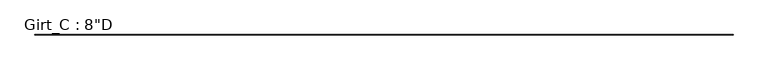
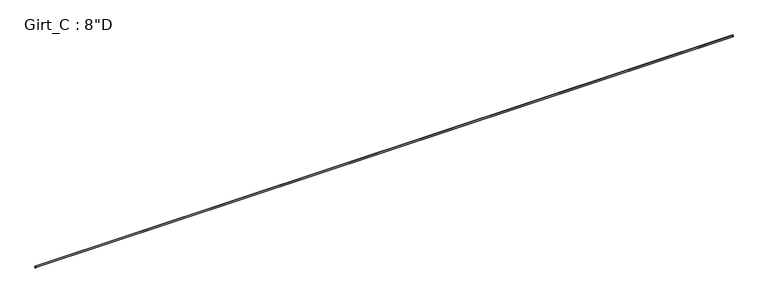
"""IFC4 building model written with IfcOpenShell, lengths in millimetres: beam geometry."""

from ifc_helpers import new_model, si_unit, point, frame, frame_2d, origin, place, context, project, spatial, polyline, circle_curve, trimmed, segment, composite_curve, outline, extrude, source, transform, mapped, element, save


def beam_1fd13926(model_context):
    return source(origin(), model_context, "Body", "SweptSolid", [
        extrude(outline(composite_curve([segment(polyline([(63.5, 101.6), (75.745104, 87.0068534), (73.6169367, 85.221109), (62.204539, 98.821875), (3.3005807, 98.821875)]), True, "CONTINUOUS"), segment(trimmed(circle_curve(frame_2d((3.3741066, 96.8381931)), 1.9850441), [point((3.3005807, 98.821875))], [point((1.3890625, 96.8381931))], True, "CARTESIAN"), True, "CONTINUOUS"), segment(polyline([(1.3890625, 96.8381931), (1.3890625, -96.8389339)]), True, "CONTINUOUS"), segment(trimmed(circle_curve(frame_2d((3.3748024, -96.8389339)), 1.9857399), [point((1.3890625, -96.8389339))], [point((3.2694106, -98.821875))], True, "CARTESIAN"), True, "CONTINUOUS"), segment(polyline([(3.2694106, -98.821875), (62.204539, -98.821875), (73.6169367, -85.221109), (75.745104, -87.0068534), (63.5, -101.6), (3.3734375, -101.6)]), True, "CONTINUOUS"), segment(trimmed(circle_curve(frame_2d((3.3734375, -96.8375)), 4.7625), [point((3.3734375, -101.6))], [point((-1.3890625, -96.8375))], False, "CARTESIAN"), True, "CONTINUOUS"), segment(polyline([(-1.3890625, -96.8375), (-1.3890625, 96.8375)]), True, "CONTINUOUS"), segment(trimmed(circle_curve(frame_2d((3.3734375, 96.8375)), 4.7625), [point((-1.3890625, 96.8375))], [point((3.3734375, 101.6))], False, "CARTESIAN"), True, "CONTINUOUS"), segment(polyline([(3.3734375, 101.6), (63.5, 101.6)]), True, "CONTINUOUS")], self_intersect=False)), frame((-45732.7, 0.0, 0.0), z_axis=(1.0, 0.0, 0.0), x_axis=(0.0, 1.0, 0.0)), (0.0, 0.0, 1.0), 91465.4),
    ])


if __name__ == "__main__":
    model = new_model("IFC4")
    model_context = context("Model", 3, world=origin())
    ifc_project = project(units=[si_unit("LENGTHUNIT", "METRE", prefix="MILLI")], contexts=[model_context])
    site = spatial("IfcSite", under=ifc_project)
    building = spatial("IfcBuilding", under=site)
    placement = place(None, origin())
    beam_shape = beam_1fd13926(model_context)
    element("IfcBeam", 1, ObjectType="Girt_C : 8\"D", at=placement, inside=building, context=model_context, shape_type="MappedRepresentation", body=[
        mapped(beam_shape, transform((0.0, 0.0, 0.0), x_axis=(1.0, 0.0, 0.0), y_axis=(0.0, 1.0, 0.0), z_axis=(0.0, 0.0, 1.0))),
    ])
    save(model, "model.ifc")

# Revit data of these elements
# Type "Girt_C : 8\"D"
#   Web_Thickness = 0' - 0 7/64"
#   Length [instance default] = 10' - 0"
#   Leg_1 = 0' - 2 1/2"
#   Height = 0' - 8"
#   Structural Material [instance default] = none
# Element 1 (IfcBeam, "Girt_C : 8\"D")
#   Structural Material = Steel
#   Materials on its faces: "Steel"
# Materials
#   "Steel": class "Metal", colour RGB 118 118 114, transparency 0, Description = "Steel, mill finish", Cost = 0
